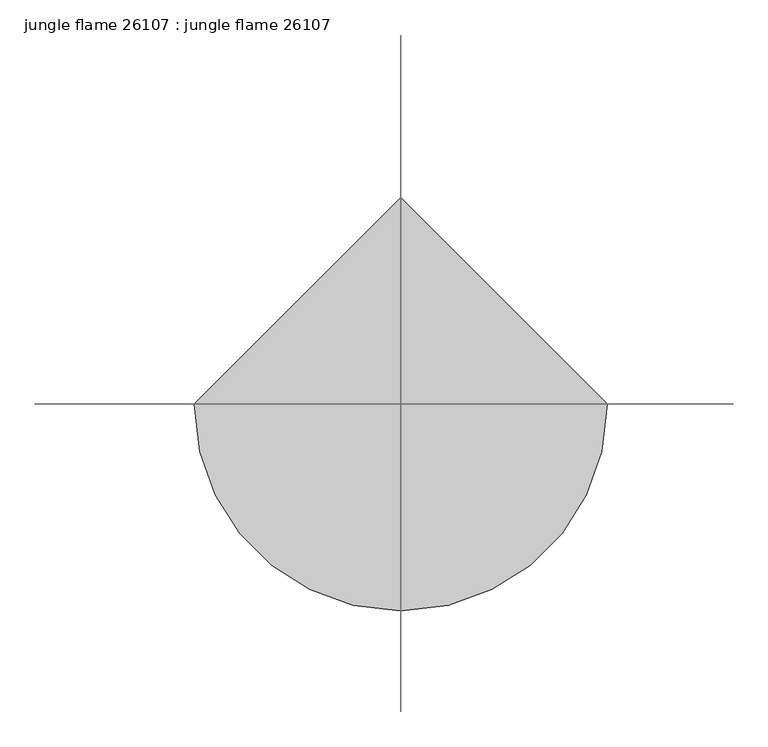
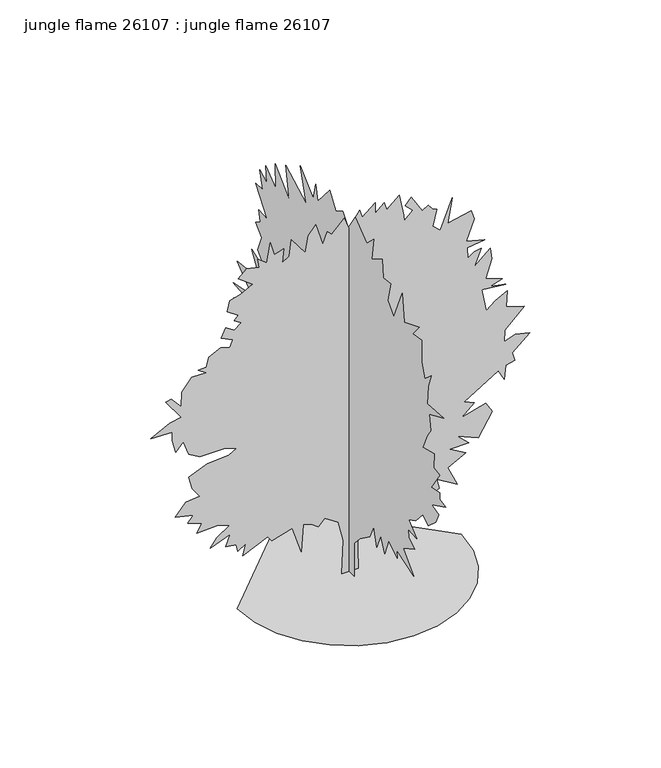
"""IFC4 building model written with IfcOpenShell, lengths in millimetres: proxy geometry, jungle flame 26107 : jungle flame 26107."""

from ifc_helpers import new_model, si_unit, origin, place, context, project, spatial, triangles, source, transform, mapped, element, save


def jungle_flame_26107_jungle_flame_26107_31e44138(model_context):
    return source(origin(), model_context, "Body", "Tessellation", [
        triangles([(-297.8835799, 0.0, 5.16e-05), (-290.0095692, -68.2551316, 5.16e-05), (-267.5813779, -130.9367389, 5.16e-05), (-232.3950082, -186.2485517, 5.16e-05), (-186.2485517, -232.3952625, 5.16e-05), (-130.9367389, -267.5813779, 5.16e-05), (-68.2551316, -290.0095692, 5.16e-05), (1.3e-05, -297.8835799, 5.16e-05), (68.2551316, -290.0095692, 5.16e-05), (130.9367389, -267.5813779, 5.16e-05), (186.2485517, -232.3950082, 5.16e-05), (232.3952625, -186.2485517, 5.16e-05), (267.5813779, -130.9367389, 5.16e-05), (290.0095692, -68.2551316, 5.16e-05), (297.8835799, 2.6e-05, 5.16e-05), (-3.91e-05, 297.8835799, 5.16e-05), (-1.65e-05, -22.3446072, 4.98e-05), (-1.37e-05, -22.4089451, 93.4481205), (-1.4e-05, -48.2564431, 121.2837307), (-1.51e-05, -93.9863508, 155.0842657), (-1.48e-05, -113.868958, 194.849244), (-1.69e-05, -127.7866314, 145.1429666), (-1.64e-05, -145.6809334, 188.8845644), (-1.84e-05, -163.5752263, 149.1193318), (-1.77e-05, -181.4695374, 196.8375492), (-2.03e-05, -221.2347519, 170.9902534), (-1.95e-05, -219.2464467, 192.8611749), (-2.38e-05, -296.7888247, 167.0136247), (-2.02e-05, -249.070353, 216.7201655), (-2.16e-05, -300.7639273, 244.5557666), (-1.99e-05, -272.9306153, 260.4617543), (-1.92e-05, -270.9418014, 282.3336933), (-2.1e-05, -310.7054898, 280.3448793), (-1.85e-05, -274.9168858, 312.1558373), (-1.94e-05, -306.7304054, 328.0638416), (-1.98e-05, -338.5413634, 363.8524638), (-2.13e-05, -364.3884049, 349.9332553), (-2.2e-05, -398.1907022, 379.7579247), (-2.17e-05, -412.1073672, 409.5800869), (-2e-05, -380.2964092, 417.5353426), (-2.19e-05, -443.9208687, 449.3463006), (-2.05e-05, -416.0849951, 455.3102171), (-2e-05, -416.0849951, 473.2045464), (-1.85e-05, -378.3075771, 465.2517978), (-1.85e-05, -416.0849951, 522.9123407), (-1.71e-05, -388.2491578, 526.8874251), (-1.6e-05, -390.2379536, 566.6536752), (-1.41e-05, -338.5413634, 554.7232987), (-1.37e-05, -358.4244884, 598.4646332), (-1.37e-05, -374.3299493, 622.325386), (-1.22e-05, -368.3660328, 664.0779247), (-1.42e-05, -433.9793243, 693.9025578), (-1.1e-05, -358.4244884, 687.9386776), (-9.7e-06, -364.3884049, 741.6215927), (-9.1e-06, -376.3187814, 777.4101786), (-8.6e-06, -346.4940757, 751.5605936), (-6.8e-06, -332.5774469, 789.3380116), (-5e-06, -332.5774469, 850.9736389), (-3.4e-06, -292.8111969, 845.0096861), (-3.7e-06, -322.6358663, 880.7983446), (-1.4e-06, -253.0469816, 852.962471), (1.3e-06, -243.1056735, 928.5173069), (3e-07, -205.3287642, 839.0458059), (2.5e-06, -177.4931631, 868.8679682), (3.5e-06, -191.4108456, 924.5396427), (4.9e-06, -157.6105468, 920.564522), (6.6e-06, -151.6456129, 968.2810135), (7.9e-06, -103.9276498, 940.4451399), (9.3e-06, -111.8806437, 1000.0944786), (9.9e-06, -80.0684139, 970.2698456), (1.34e-05, -28.3738313, 1012.0223116), (1.33e-05, 3.4383978, 962.3170607), (1.55e-05, 29.285692, 994.128055), (1.63e-05, 61.0979195, 976.2337257), (1.88e-05, 88.9335251, 1015.9999758), (1.94e-05, 144.6047364, 952.3755163), (2.1e-05, 154.5460354, 994.128055), (2.02e-05, 166.475667, 946.4115635), (2.45e-05, 226.1232435, 1002.0833107), (2.06e-05, 198.2876424, 912.6118097), (2.63e-05, 291.7367712, 964.3058928), (2.3e-05, 275.8287488, 876.8232239), (2.77e-05, 339.4532264, 938.4588512), (2.56e-05, 337.4669377, 870.8567276), (2.87e-05, 383.1945608, 906.6453861), (2.71e-05, 379.2194401, 860.9151833), (2.91e-05, 411.0303981, 878.8095125), (2.7e-05, 397.113733, 831.0930937), (2.85e-05, 430.9135231, 829.1042616), (2.4e-05, 377.2306443, 759.5158493), (2.58e-05, 415.0080623, 763.49097), (2.47e-05, 409.0441458, 733.6662643), (2.52e-05, 430.9135231, 719.7495993), (2.32e-05, 403.0776858, 691.9137983), (2.26e-05, 420.9719788, 648.1724276), (1.97e-05, 381.2082722, 608.4061775), (2.34e-05, 448.807816, 632.2669304), (1.9e-05, 401.0888537, 554.7232987), (2.1e-05, 436.8774396, 568.6424709), (2.42e-05, 514.4211076, 558.7009266), (1.96e-05, 448.807816, 505.0180115), (2.28e-05, 532.3154005, 487.1237185), (1.85e-05, 440.8551038, 479.1710063), (1.74e-05, 430.9135231, 457.2990492), (2.16e-05, 530.3266047, 447.3575048), (1.66e-05, 438.8662717, 419.5216312), (1.6e-05, 456.7605646, 369.8163803), (1.51e-05, 409.0441458, 411.5688827), (1.33e-05, 395.1249372, 371.8051761), (1.47e-05, 442.8438995, 349.9332553), (1.34e-05, 444.8327316, 302.2142748), (9.7e-06, 379.2194401, 276.3672333), (1.12e-05, 426.9384387, 254.4978378), (5.4e-06, 323.5477292, 216.7201655), (7.3e-06, 379.2194401, 194.849244), (7.4e-06, 411.0303981, 151.1076461), (4.7e-06, 327.5253571, 184.9081902), (2.9e-06, 321.5588971, 135.2016584), (2.6e-06, 287.7591252, 174.966882), (0.0, 265.8897297, 119.2956707), (1.8e-06, 267.8760183, 176.9549329), (1.3e-06, 253.9588446, 182.9198668), (-1.2e-06, 226.1232435, 141.1663379), (-2e-07, 228.1115487, 170.9902534), (-2.1e-06, 180.3933313, 176.9549329), (-2.7e-06, 186.3580108, 151.1076461), (-3.4e-06, 154.5460354, 174.966882), (-6.1e-06, 144.6047364, 99.4130544), (-6.1e-06, 82.9688456, 190.8728697), (-7.1e-06, 69.0509133, 178.9432563), (-8.2e-06, 41.2153077, 182.9198668), (-8.5e-06, 57.1215497, 149.1193318), (-9.5e-06, 17.3562001, 174.966882), (-1.44e-05, 25.309295, 5.13e-05), (-19.2607679, 5.89e-05, 1.9e-06), (-15.3064967, 5.32e-05, 92.9241154), (-29.1462451, 5.05e-05, 148.2829094), (-64.7341846, 5.06e-05, 172.0082871), (-82.5281566, 5.25e-05, 154.2143151), (-100.3221195, 5.24e-05, 168.0540227), (-122.0703651, 5.3e-05, 173.9854194), (-128.0015165, 5.76e-05, 100.8324082), (-151.7268943, 5.43e-05, 173.9854194), (-205.1088103, 5.76e-05, 158.1685977), (-216.9713675, 5.72e-05, 173.9854194), (-282.2168581, 6.19e-05, 142.351758), (-274.3072937, 5.97e-05, 173.9854194), (-296.0547671, 6.15e-05, 160.14573), (-300.0095584, 6.05e-05, 179.9165799), (-327.6904633, 6.14e-05, 183.8708443), (-315.8261438, 5.9e-05, 215.5045239), (-369.2092953, 6.27e-05, 193.7565236), (-351.4140879, 6.05e-05, 217.4816561), (-317.8048021, 5.76e-05, 241.2070248), (-351.4140879, 5.85e-05, 251.0924498), (-404.7972393, 6.09e-05, 249.1153175), (-390.956805, 5.9e-05, 270.8630453), (-428.5208639, 5.98e-05, 284.7035159), (-414.6829368, 5.82e-05, 302.4962162), (-462.1326568, 5.95e-05, 314.3605356), (-434.4542953, 5.64e-05, 345.9937065), (-396.887693, 5.46e-05, 349.9484797), (-416.6590516, 5.38e-05, 377.6268774), (-426.5447127, 5.21e-05, 413.2148214), (-377.1163344, 4.86e-05, 434.9622949), (-319.780917, 4.59e-05, 438.917068), (-298.0334254, 4.42e-05, 450.7814238), (-333.6213876, 4.52e-05, 460.6645414), (-396.887693, 4.8e-05, 460.6645414), (-426.5447127, 4.82e-05, 478.4597852), (-440.3851833, 4.64e-05, 518.0025023), (-460.1565419, 4.86e-05, 496.2524855), (-470.0396959, 4.69e-05, 531.8404295), (-470.0396959, 4.55e-05, 555.5665612), (-527.3776568, 4.79e-05, 557.5426761), (-475.9731274, 4.41e-05, 583.2475024), (-446.3160713, 4.25e-05, 589.1783904), (-487.8349397, 4.09e-05, 646.5138079), (-472.0183542, 4e-05, 648.4899227), (-446.3160713, 4.07e-05, 618.8354101), (-444.337413, 3.82e-05, 658.3755838), (-418.6351665, 3.51e-05, 691.987413), (-379.0949927, 3.35e-05, 690.0087547), (-400.8424662, 3.35e-05, 705.8278473), (-379.0949927, 3.26e-05, 705.8278473), (-373.1615613, 3.08e-05, 731.5301302), (-341.5283904, 2.84e-05, 747.346752), (-317.8048021, 2.79e-05, 739.437133), (-309.8952195, 2.64e-05, 759.2085279), (-339.5522756, 2.68e-05, 773.0489622), (-327.6904633, 2.48e-05, 798.7512451), (-305.9404464, 2.47e-05, 784.9108109), (-286.1690878, 2.3e-05, 798.7512451), (-305.9404464, 2.31e-05, 810.6130211), (-294.0786522, 2.19e-05, 822.4748697), (-323.7356901, 2.2e-05, 842.246192), (-317.8048021, 2e-05, 871.903248), (-288.1477461, 1.82e-05, 879.8127943), (-256.5145934, 1.59e-05, 895.6293434), (-294.0786522, 1.58e-05, 925.2863995), (-272.3311788, 1.36e-05, 945.0577944), (-238.719604, 1.26e-05, 937.1482481), (-242.6736322, 1.14e-05, 960.8743435), (-218.9484997, 1.14e-05, 943.0791361), (-209.0628204, 7.8e-06, 996.4622875), (-199.1773955, 9.6e-06, 958.8956852), (-173.4748764, 8e-06, 966.8052315), (-177.429159, 1.04e-05, 929.2386292), (-159.635187, 8.9e-06, 941.1030212), (-153.7037722, 6.1e-06, 984.5979681), (-116.1389593, 7.4e-06, 935.1721333), (-108.2304123, 4.3e-06, 980.6457384), (-88.459308, 2.1e-06, 1004.3692904), (-70.6655904, 4.9e-06, 943.0791361), (-58.8027788, 2.5e-06, 974.712307), (-46.9402171, 2.7e-06, 962.8504583), (-13.329386, -7e-07, 996.4622875), (-1.4667204, 6e-07, 964.8265732), (28.1899354, -3e-06, 1004.3692904), (34.1210891, -2e-06, 982.6218533), (69.7090263, -5.2e-06, 1010.300251), (69.7090263, -3.4e-06, 980.6457384), (93.4344041, -5.8e-06, 1002.3931755), (99.3655555, -4.7e-06, 980.6457384), (132.9763673, -8e-06, 1010.300251), (144.8391788, -4.8e-06, 949.0100241), (146.816311, -4e-06, 933.1934023), (168.5642931, -6.2e-06, 954.9434555), (148.793198, -6.5e-06, 974.712307), (164.610283, -8.3e-06, 992.5075144), (194.2668122, -6.8e-06, 945.0577944), (210.083652, -8e-06, 954.9434555), (219.969077, -7.6e-06, 941.1030212), (231.8318885, -7.8e-06, 935.1721333), (221.9462092, -4.8e-06, 891.6745703), (241.7173134, -4.6e-06, 873.8819063), (273.3497213, -1.07e-05, 952.9647972), (261.487909, -6.2e-06, 885.7436823), (324.756776, -9.8e-06, 899.5841892), (332.6637789, -8.6e-06, 873.8819063), (310.9163054, -4.3e-06, 818.5225674), (360.3447201, -5.7e-06, 804.6821331), (312.8924203, -3.2e-06, 798.7512451), (314.8710786, -1.5e-06, 769.0941891), (332.6637789, -3e-06, 780.9560377), (350.4590226, -4e-06, 784.9108109), (332.6637789, -6e-07, 739.437133), (374.1826472, -4.6e-06, 777.0037354), (378.1374204, -2.9e-06, 745.3680937), (362.3208349, 7e-07, 695.9421862), (405.8183252, -2e-07, 680.1256371), (374.1826472, 1.8e-06, 670.2399759), (415.7014792, 5e-07, 660.3542421), (352.4351375, 2.8e-06, 668.2613176), (364.2969498, 6.1e-06, 604.9949759), (388.0230815, 3.9e-06, 624.7662981), (419.6562524, 1.5e-06, 640.5829199), (417.6801375, 4.2e-06, 597.0853932), (465.1298575, 3.1e-06, 581.2688441), (413.7253644, 8.3e-06, 531.8404295), (411.7492132, 1.02e-05, 500.2072586), (441.4037258, 8.2e-06, 512.0716144), (478.9703281, 7.2e-06, 502.1859169), (433.496723, 1.15e-05, 462.6431997), (439.427611, 1.27e-05, 438.917068), (415.7014792, 1.41e-05, 432.98618), (411.7492132, 1.65e-05, 395.4221211), (395.9326641, 1.54e-05, 425.0765974), (304.9854175, 2.27e-05, 369.7198382), (332.6637789, 2.22e-05, 357.8555188), (297.075853, 2.55e-05, 328.1984628), (362.3208349, 2.16e-05, 345.9937065), (380.1135352, 2.26e-05, 316.3366868), (342.5494763, 2.79e-05, 255.046478), (287.1901737, 2.89e-05, 278.7726098), (316.8472298, 2.92e-05, 251.0924498), (267.4188151, 3.15e-05, 249.1153175), (308.9376472, 3.11e-05, 225.3902032), (261.487909, 3.47e-05, 199.6876841), (287.1901737, 3.69e-05, 144.3286358), (231.8316341, 3.73e-05, 177.9394476), (239.7401812, 3.86e-05, 150.2600507), (200.1979727, 4.14e-05, 132.4660787), (162.6331508, 4.11e-05, 166.0768723), (168.5642931, 4.56e-05, 85.0155775), (146.816311, 4.22e-05, 158.1685977), (91.4572718, 4.73e-05, 112.6949744), (101.3426968, 4.41e-05, 160.14573), (59.8236013, 4.92e-05, 104.7866817), (47.9607853, 4.76e-05, 140.3746166), (73.6632998, 4.26e-05, 205.6190989), (38.0753603, 4.45e-05, 199.6876841), (20.2813656, 4.7e-05, 170.0311549), (24.2355619, 5.7e-05, 0.0)], [[15, 16, 1], [14, 15, 1], [14, 1, 2], [13, 14, 2], [13, 2, 3], [13, 3, 4], [12, 13, 4], [11, 12, 4], [11, 4, 5], [11, 5, 6], [11, 6, 7], [11, 7, 8], [11, 8, 9], [11, 9, 10], [101, 102, 103], [119, 120, 121], [51, 52, 53], [104, 105, 106], [76, 77, 78], [27, 28, 29], [59, 60, 61], [106, 107, 108], [78, 79, 80], [122, 123, 124], [61, 62, 63], [54, 55, 56], [131, 132, 133], [115, 116, 117], [114, 115, 117], [21, 22, 23], [40, 41, 42], [32, 33, 34], [96, 97, 98], [68, 69, 70], [125, 126, 127], [127, 128, 129], [82, 83, 84], [86, 87, 88], [112, 113, 114], [23, 24, 25], [99, 100, 101], [84, 85, 86], [117, 118, 119], [80, 81, 82], [25, 26, 27], [88, 89, 90], [29, 30, 31], [44, 45, 46], [66, 67, 68], [64, 65, 66], [90, 91, 92], [46, 47, 48], [74, 75, 76], [92, 93, 94], [42, 43, 44], [40, 42, 44], [38, 39, 40], [98, 99, 101], [57, 58, 59], [70, 71, 72], [133, 134, 17], [133, 17, 18], [133, 18, 19], [104, 106, 108], [114, 117, 119], [72, 73, 74], [133, 19, 20], [37, 38, 40], [36, 37, 40], [133, 20, 21], [110, 111, 112], [109, 110, 112], [44, 46, 48], [53, 54, 56], [94, 95, 96], [98, 101, 103], [90, 92, 94], [68, 70, 72], [114, 119, 121], [114, 121, 122], [98, 103, 104], [129, 130, 131], [64, 66, 68], [86, 88, 90], [84, 86, 90], [82, 84, 90], [25, 27, 29], [25, 29, 31], [25, 31, 32], [57, 59, 61], [57, 61, 63], [56, 57, 63], [53, 56, 63], [98, 104, 108], [49, 50, 51], [36, 40, 44], [36, 44, 48], [35, 36, 48], [34, 35, 48], [25, 32, 34], [23, 25, 34], [21, 23, 34], [21, 34, 48], [133, 21, 48], [131, 133, 48], [129, 131, 48], [90, 94, 96], [82, 90, 96], [80, 82, 96], [109, 112, 114], [109, 114, 122], [64, 68, 72], [122, 124, 125], [109, 122, 125], [109, 125, 127], [109, 127, 129], [109, 129, 48], [108, 109, 48], [98, 108, 48], [96, 98, 48], [80, 96, 48], [78, 80, 48], [76, 78, 48], [74, 76, 48], [72, 74, 48], [64, 72, 48], [63, 64, 48], [53, 63, 48], [53, 48, 49], [53, 49, 51], [252, 253, 254], [236, 237, 238], [284, 285, 286], [141, 142, 143], [241, 242, 243], [204, 205, 206], [174, 175, 176], [151, 152, 153], [279, 280, 281], [266, 267, 268], [183, 184, 185], [250, 251, 252], [151, 153, 154], [286, 287, 288], [202, 203, 204], [209, 210, 211], [275, 276, 277], [145, 146, 147], [218, 219, 220], [220, 221, 222], [247, 248, 249], [288, 289, 290], [288, 290, 291], [155, 156, 157], [262, 263, 264], [212, 213, 214], [211, 212, 214], [245, 246, 247], [244, 245, 247], [171, 172, 173], [277, 278, 279], [261, 262, 264], [224, 225, 226], [256, 257, 258], [177, 178, 179], [177, 179, 180], [258, 259, 260], [222, 223, 224], [159, 160, 161], [269, 270, 271], [247, 249, 250], [216, 217, 218], [214, 215, 216], [206, 207, 208], [147, 148, 149], [250, 252, 254], [159, 161, 162], [157, 158, 159], [229, 230, 231], [228, 229, 231], [193, 194, 195], [149, 150, 151], [199, 200, 201], [199, 201, 202], [190, 191, 192], [189, 190, 192], [294, 135, 136], [293, 294, 136], [293, 136, 137], [204, 206, 208], [174, 176, 177], [264, 265, 266], [231, 232, 233], [238, 239, 240], [238, 240, 241], [236, 238, 241], [138, 139, 140], [255, 256, 258], [255, 258, 260], [163, 164, 165], [281, 282, 283], [281, 283, 284], [273, 274, 275], [272, 273, 275], [271, 272, 275], [233, 234, 235], [231, 233, 235], [162, 163, 165], [162, 165, 166], [143, 144, 145], [195, 196, 197], [195, 197, 198], [227, 228, 231], [227, 231, 235], [171, 173, 174], [171, 174, 177], [261, 264, 266], [261, 266, 268], [195, 198, 199], [293, 137, 138], [292, 293, 138], [157, 159, 162], [155, 157, 162], [155, 162, 166], [154, 155, 166], [154, 166, 167], [286, 288, 291], [284, 286, 291], [181, 182, 183], [180, 181, 183], [247, 250, 254], [147, 149, 151], [185, 186, 187], [185, 187, 188], [183, 185, 188], [199, 202, 204], [199, 204, 208], [224, 226, 227], [277, 279, 281], [277, 281, 284], [277, 284, 291], [261, 268, 269], [189, 192, 193], [236, 241, 243], [193, 195, 199], [193, 199, 208], [145, 147, 151], [145, 151, 154], [145, 154, 167], [143, 145, 167], [141, 143, 167], [222, 224, 227], [275, 277, 291], [271, 275, 291], [269, 271, 291], [177, 180, 183], [140, 141, 167], [138, 140, 167], [292, 138, 167], [291, 292, 167], [269, 291, 167], [261, 269, 167], [260, 261, 167], [255, 260, 167], [254, 255, 167], [247, 254, 167], [244, 247, 167], [243, 244, 167], [236, 243, 167], [235, 236, 167], [227, 235, 167], [222, 227, 167], [220, 222, 167], [218, 220, 167], [216, 218, 167], [214, 216, 167], [211, 214, 167], [209, 211, 167], [208, 209, 167], [193, 208, 167], [189, 193, 167], [188, 189, 167], [183, 188, 167], [177, 183, 167], [177, 167, 168], [171, 177, 168], [171, 168, 169], [170, 171, 169]], closed=False),
    ])


if __name__ == "__main__":
    model = new_model("IFC4")
    model_context = context("Model", 3, world=origin())
    ifc_project = project(units=[si_unit("LENGTHUNIT", "METRE", prefix="MILLI")], contexts=[model_context])
    site = spatial("IfcSite", under=ifc_project)
    building = spatial("IfcBuilding", under=site)
    placement = place(None, origin())
    jungle_flame_26107_jungle_flame_26107_shape = jungle_flame_26107_jungle_flame_26107_31e44138(model_context)
    element("IfcBuildingElementProxy", 1, Name="jungle flame 26107 : jungle flame 26107", ObjectType="jungle flame 26107 : jungle flame 26107", at=placement, inside=building, context=model_context, shape_type="MappedRepresentation", body=[
        mapped(jungle_flame_26107_jungle_flame_26107_shape, transform((0.0, 0.0, 0.0), x_axis=(1.0, 0.0, 0.0), y_axis=(0.0, 1.0, 0.0), z_axis=(0.0, 0.0, 1.0))),
    ])
    save(model, "model.ifc")

# Revit data of these elements
# Type "jungle flame 26107 : jungle flame 26107"
#   built-in parameter 1005195 = "RPC-16-FUVJ-JWG0-MWGK-8000-ST1L-LVER-AU"
#   Height = 0
